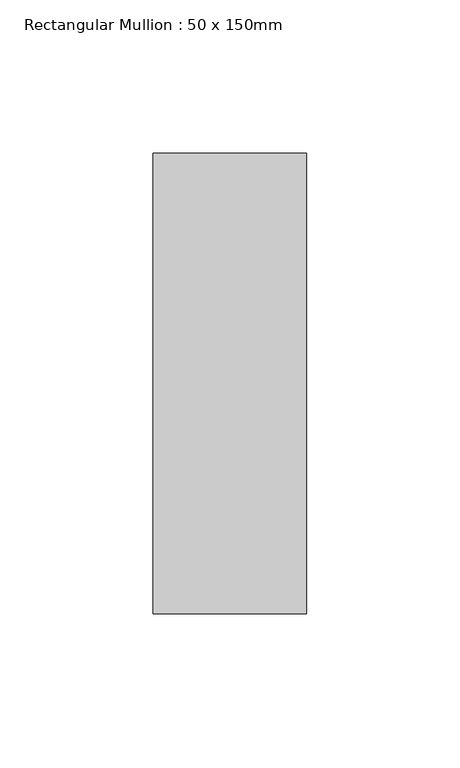
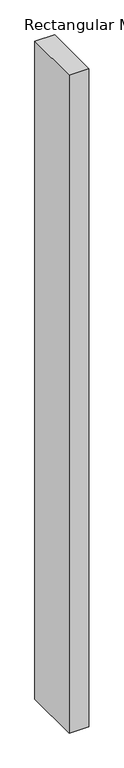
"""IFC4 building model written with IfcOpenShell, lengths in millimetres: member geometry, Rectangular Mullion : 50 x 150mm."""

import ifcopenshell
import ifcopenshell.guid

model = None  # the IFC model being written
_history = None  # IfcOwnerHistory: only IFC2X3 demands one
_inside = {}  # id of a spatial element -> (the spatial element, [elements in it])
_under = {}  # id of a project, library or spatial element -> (it, [spatial elements below it])
_declared = {}  # id of a project -> (the project, [libraries it declares])
_typed = {}  # id of a type object -> (the type object, [elements of that type])
_made_of = {}  # id of a material, layer set ... -> (it, [elements and type objects made of it])


def new_model(schema):
    """Start an empty IFC model of exactly this schema.

    Asked for "IFC4X3", IfcOpenShell would pick the latest addendum, in which some entities
    have other attributes; the version numbers below select the first issue.
    IFC2X3 requires an IfcOwnerHistory on every rooted entity: one is made here for all.
    """
    global model, _history
    if schema == "IFC4X3":
        model = ifcopenshell.file(schema_version=(4, 3, 0, 0))
    else:
        model = ifcopenshell.file(schema=schema)
    _inside.clear()
    _under.clear()
    _declared.clear()
    _typed.clear()
    _made_of.clear()
    _history = None
    if model.schema == "IFC2X3":
        org = make("IfcOrganization", Name="unknown")
        user = make(
            "IfcPersonAndOrganization",
            ThePerson=make("IfcPerson", FamilyName="unknown"),
            TheOrganization=org,
        )
        app = make(
            "IfcApplication",
            ApplicationDeveloper=org,
            Version="unknown",
            ApplicationFullName="unknown",
            ApplicationIdentifier="unknown",
        )
        _history = make(
            "IfcOwnerHistory",
            OwningUser=user,
            OwningApplication=app,
            ChangeAction="ADDED",
            CreationDate=0,
        )
    return model


def make(cls, **values):
    """One entity of the class cls with the attributes given. An attribute that is None is left unset."""
    return model.create_entity(
        cls, **{name: value for name, value in values.items() if value is not None}
    )


def rooted(cls, **values):
    """An entity with a GlobalId (a new one), such as an element, a storey or a relation."""
    return make(cls, GlobalId=ifcopenshell.guid.new(), OwnerHistory=_history, **values)


def si_unit(unit_type, name, prefix=None):
    """IfcSIUnit, for example si_unit("LENGTHUNIT", "METRE", prefix="MILLI")."""
    return make("IfcSIUnit", UnitType=unit_type, Prefix=prefix, Name=name)


def assignment(units):
    """IfcUnitAssignment: the units of a project."""
    return None if units is None else make("IfcUnitAssignment", Units=units)


def point(xyz):
    """IfcCartesianPoint."""
    return None if xyz is None else make("IfcCartesianPoint", Coordinates=xyz)


def direction(xyz):
    """IfcDirection."""
    return None if xyz is None else make("IfcDirection", DirectionRatios=xyz)


def frame(location, z_axis=None, x_axis=None):
    """IfcAxis2Placement3D, a coordinate frame: its origin and axes. An axis left out is left unset."""
    return make(
        "IfcAxis2Placement3D",
        Location=point(location),
        Axis=direction(z_axis),
        RefDirection=direction(x_axis),
    )


def origin():
    """The frame at (0, 0, 0) with its axes left unset."""
    return frame((0.0, 0.0, 0.0))


def place(relative_to, where):
    """IfcLocalPlacement: puts the frame where relative to a parent placement (None: the world)."""
    return make(
        "IfcLocalPlacement", PlacementRelTo=relative_to, RelativePlacement=where
    )


def context(
    kind, dimensions, precision=None, world=None, true_north=None, identifier=None
):
    """IfcGeometricRepresentationContext, for example the 3D "Model" context."""
    return make(
        "IfcGeometricRepresentationContext",
        ContextIdentifier=identifier,
        ContextType=kind,
        CoordinateSpaceDimension=dimensions,
        Precision=precision,
        WorldCoordinateSystem=world,
        TrueNorth=true_north,
    )


def project(units=None, contexts=None):
    """IfcProject with its units and contexts."""
    return rooted(
        "IfcProject",
        Name="project",
        RepresentationContexts=contexts,
        UnitsInContext=assignment(units),
    )


def spatial(cls, under=None, at=None, **own):
    """A site, building, storey or space (cls), placed at a placement, below another one or the project."""
    s = rooted(cls, ObjectPlacement=at, **own)
    if under is not None:
        _under.setdefault(under.id(), (under, []))[1].append(s)
    return s


def polyline(points):
    """IfcPolyline through the points."""
    return make("IfcPolyline", Points=[point(p) for p in points])


def outline(outer, holes=None, kind="AREA"):
    """IfcArbitraryClosedProfileDef: a profile drawn as a closed curve; with holes, ...WithVoids."""
    if holes is None:
        return make("IfcArbitraryClosedProfileDef", ProfileType=kind, OuterCurve=outer)
    return make(
        "IfcArbitraryProfileDefWithVoids",
        ProfileType=kind,
        OuterCurve=outer,
        InnerCurves=holes,
    )


def extrude(swept, where, along, depth):
    """IfcExtrudedAreaSolid: the profile swept, set in the frame where, extruded along a direction by depth."""
    return make(
        "IfcExtrudedAreaSolid",
        SweptArea=swept,
        Position=where,
        ExtrudedDirection=direction(along),
        Depth=depth,
    )


def shape(context_of_items, identifier, shape_type, items):
    """IfcShapeRepresentation: the items that make up one representation, for example the "Body"."""
    return make(
        "IfcShapeRepresentation",
        ContextOfItems=context_of_items,
        RepresentationIdentifier=identifier,
        RepresentationType=shape_type,
        Items=items,
    )


def source(mapping_origin, context_of_items, identifier, shape_type, items):
    """IfcRepresentationMap: a shape defined once, which mapped items show again and again."""
    return make(
        "IfcRepresentationMap",
        MappingOrigin=mapping_origin,
        MappedRepresentation=shape(context_of_items, identifier, shape_type, items),
    )


def transform(
    local_origin,
    x_axis=None,
    y_axis=None,
    z_axis=None,
    scale=None,
    scale2=None,
    scale3=None,
    uniform=True,
):
    """IfcCartesianTransformationOperator3D, or its non-uniform kind. x_axis, y_axis, z_axis: its Axis1, 2, 3."""
    if uniform:
        return make(
            "IfcCartesianTransformationOperator3D",
            Axis1=direction(x_axis),
            Axis2=direction(y_axis),
            LocalOrigin=point(local_origin),
            Scale=scale,
            Axis3=direction(z_axis),
        )
    return make(
        "IfcCartesianTransformationOperator3DnonUniform",
        Axis1=direction(x_axis),
        Axis2=direction(y_axis),
        LocalOrigin=point(local_origin),
        Scale=scale,
        Axis3=direction(z_axis),
        Scale2=scale2,
        Scale3=scale3,
    )


def mapped(mapping_source, mapping_target):
    """IfcMappedItem: shows the shape of a source again, moved by a transform."""
    return make(
        "IfcMappedItem", MappingSource=mapping_source, MappingTarget=mapping_target
    )


def made_of(thing, what):
    """Note that an element or type object is made of a material, layer set ...; save() writes the relation."""
    if what is not None:
        _made_of.setdefault(what.id(), (what, []))[1].append(thing)
    return thing


def element(
    cls,
    number,
    at=None,
    inside=None,
    cuts=None,
    type_object=None,
    material=None,
    context=None,
    identifier="Body",
    shape_type=None,
    held_by="IfcProductDefinitionShape",
    body=None,
    shapes=None,
    **own,
):
    """One element of the class cls, such as IfcWall. Its Tag is "e" and its number.

    at: its placement. inside: the storey or other place that contains it. cuts: it is an
    opening in that element (IfcRelVoidsElement). A single representation is given by context,
    identifier, shape_type and body (its items); several are given by shapes. held_by: the class
    of the entity that holds the representations. save() writes the other relations.
    """
    e = rooted(cls, Tag="e%d" % number, ObjectPlacement=at, **own)
    if body is not None:
        shapes = [shape(context, identifier, shape_type, body)]
    if shapes is not None:
        e.Representation = make(held_by, Representations=shapes)
    if inside is not None:
        _inside.setdefault(inside.id(), (inside, []))[1].append(e)
    if cuts is not None:
        rooted(
            "IfcRelVoidsElement", RelatingBuildingElement=cuts, RelatedOpeningElement=e
        )
    if type_object is not None:
        _typed.setdefault(type_object.id(), (type_object, []))[1].append(e)
    return made_of(e, material)


def aggregate(whole, parts):
    """IfcRelAggregates: a whole, such as a stair, and the parts it consists of."""
    return rooted("IfcRelAggregates", RelatingObject=whole, RelatedObjects=parts)


def save(model, path):
    """Write the relations noted so far, then the file.

    IfcRelAggregates (storeys below a building ...), IfcRelContainedInSpatialStructure (elements
    in a storey), IfcRelDefinesByType, IfcRelAssociatesMaterial and IfcRelDeclares: one each for
    every whole, place, type object, material and project.
    """
    for whole, parts in _under.values():
        aggregate(whole, parts)
    for where, things in _inside.values():
        rooted(
            "IfcRelContainedInSpatialStructure",
            RelatedElements=things,
            RelatingStructure=where,
        )
    for kind, things in _typed.values():
        rooted("IfcRelDefinesByType", RelatedObjects=things, RelatingType=kind)
    for what, things in _made_of.values():
        rooted("IfcRelAssociatesMaterial", RelatedObjects=things, RelatingMaterial=what)
    for by, libraries in _declared.values():
        rooted("IfcRelDeclares", RelatingContext=by, RelatedDefinitions=libraries)
    model.write(path)


def rectangular_mullion_50_x_150mm_661033a2(model_context):
    return source(origin(), model_context, "Body", "SweptSolid", [
        extrude(outline(polyline([(0.0, 75.0), (0.0, -75.0), (-50.0, -75.0), (-50.0, 75.0), (0.0, 75.0)])), frame((0.0, 0.0, -1759.0), z_axis=(0.0, 0.0, 1.0), x_axis=(1.0, 0.0, 0.0)), (0.0, 0.0, 1.0), 1759.0),
    ])


if __name__ == "__main__":
    model = new_model("IFC4")
    model_context = context("Model", 3, world=origin())
    ifc_project = project(units=[si_unit("LENGTHUNIT", "METRE", prefix="MILLI")], contexts=[model_context])
    site = spatial("IfcSite", under=ifc_project)
    building = spatial("IfcBuilding", under=site)
    placement = place(None, origin())
    rectangular_mullion_50_x_150mm_shape = rectangular_mullion_50_x_150mm_661033a2(model_context)
    element("IfcMember", 1, ObjectType="Rectangular Mullion : 50 x 150mm", at=placement, inside=building, context=model_context, shape_type="MappedRepresentation", body=[
        mapped(rectangular_mullion_50_x_150mm_shape, transform((0.0, 0.0, 0.0), x_axis=(1.0, 0.0, 0.0), y_axis=(0.0, 1.0, 0.0), z_axis=(0.0, 0.0, 1.0))),
    ])
    save(model, "model.ifc")

# Revit data of these elements
# Type "Rectangular Mullion : 50 x 150mm"
#   Keynote = "H11"
#   built-in parameter 1007304 = 0.492126 (stored number, unit not read)
#   built-in parameter 1007301 = 0.082021 (stored number, unit not read)
#   built-in parameter 1007300 = 0.082021 (stored number, unit not read)
# Element 1 (IfcMember, "Rectangular Mullion : 50 x 150mm")
#   Materials on its faces: "Aluminium"
# Materials
#   "Aluminium": class "Metal", colour RGB 247 247 247, transparency 0, Description = "Aluminium 6061", Cost = 0
